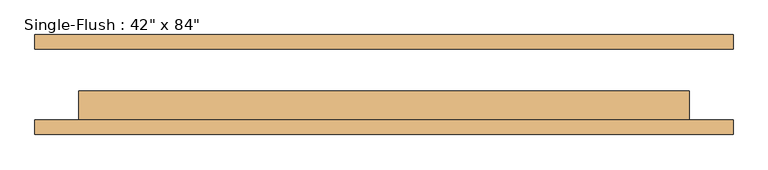
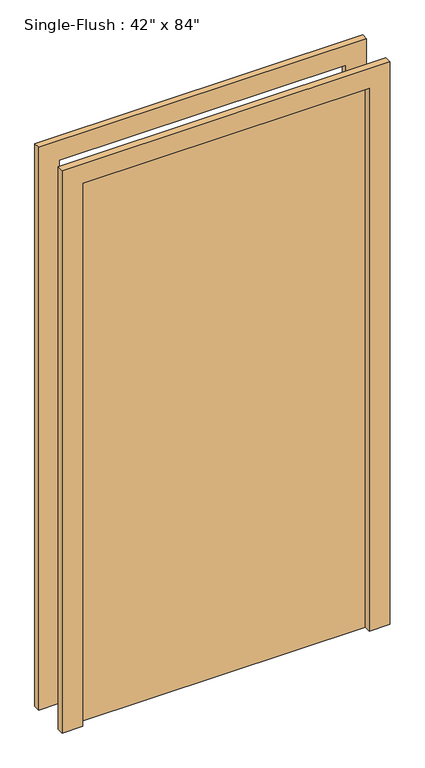
"""IFC4 building model written with IfcOpenShell, lengths in millimetres: door geometry."""

import ifcopenshell
import ifcopenshell.guid

model = None  # the IFC model being written
_history = None  # IfcOwnerHistory: only IFC2X3 demands one
_inside = {}  # id of a spatial element -> (the spatial element, [elements in it])
_under = {}  # id of a project, library or spatial element -> (it, [spatial elements below it])
_declared = {}  # id of a project -> (the project, [libraries it declares])
_typed = {}  # id of a type object -> (the type object, [elements of that type])
_made_of = {}  # id of a material, layer set ... -> (it, [elements and type objects made of it])


def new_model(schema):
    """Start an empty IFC model of exactly this schema.

    Asked for "IFC4X3", IfcOpenShell would pick the latest addendum, in which some entities
    have other attributes; the version numbers below select the first issue.
    IFC2X3 requires an IfcOwnerHistory on every rooted entity: one is made here for all.
    """
    global model, _history
    if schema == "IFC4X3":
        model = ifcopenshell.file(schema_version=(4, 3, 0, 0))
    else:
        model = ifcopenshell.file(schema=schema)
    _inside.clear()
    _under.clear()
    _declared.clear()
    _typed.clear()
    _made_of.clear()
    _history = None
    if model.schema == "IFC2X3":
        org = make("IfcOrganization", Name="unknown")
        user = make(
            "IfcPersonAndOrganization",
            ThePerson=make("IfcPerson", FamilyName="unknown"),
            TheOrganization=org,
        )
        app = make(
            "IfcApplication",
            ApplicationDeveloper=org,
            Version="unknown",
            ApplicationFullName="unknown",
            ApplicationIdentifier="unknown",
        )
        _history = make(
            "IfcOwnerHistory",
            OwningUser=user,
            OwningApplication=app,
            ChangeAction="ADDED",
            CreationDate=0,
        )
    return model


def make(cls, **values):
    """One entity of the class cls with the attributes given. An attribute that is None is left unset."""
    return model.create_entity(
        cls, **{name: value for name, value in values.items() if value is not None}
    )


def rooted(cls, **values):
    """An entity with a GlobalId (a new one), such as an element, a storey or a relation."""
    return make(cls, GlobalId=ifcopenshell.guid.new(), OwnerHistory=_history, **values)


def si_unit(unit_type, name, prefix=None):
    """IfcSIUnit, for example si_unit("LENGTHUNIT", "METRE", prefix="MILLI")."""
    return make("IfcSIUnit", UnitType=unit_type, Prefix=prefix, Name=name)


def assignment(units):
    """IfcUnitAssignment: the units of a project."""
    return None if units is None else make("IfcUnitAssignment", Units=units)


def point(xyz):
    """IfcCartesianPoint."""
    return None if xyz is None else make("IfcCartesianPoint", Coordinates=xyz)


def direction(xyz):
    """IfcDirection."""
    return None if xyz is None else make("IfcDirection", DirectionRatios=xyz)


def frame(location, z_axis=None, x_axis=None):
    """IfcAxis2Placement3D, a coordinate frame: its origin and axes. An axis left out is left unset."""
    return make(
        "IfcAxis2Placement3D",
        Location=point(location),
        Axis=direction(z_axis),
        RefDirection=direction(x_axis),
    )


def origin():
    """The frame at (0, 0, 0) with its axes left unset."""
    return frame((0.0, 0.0, 0.0))


def origin_with_axes():
    """The frame at (0, 0, 0) with the z axis (0, 0, 1) and the x axis (1, 0, 0) written out."""
    return frame((0.0, 0.0, 0.0), z_axis=(0.0, 0.0, 1.0), x_axis=(1.0, 0.0, 0.0))


def place(relative_to, where):
    """IfcLocalPlacement: puts the frame where relative to a parent placement (None: the world)."""
    return make(
        "IfcLocalPlacement", PlacementRelTo=relative_to, RelativePlacement=where
    )


def context(
    kind, dimensions, precision=None, world=None, true_north=None, identifier=None
):
    """IfcGeometricRepresentationContext, for example the 3D "Model" context."""
    return make(
        "IfcGeometricRepresentationContext",
        ContextIdentifier=identifier,
        ContextType=kind,
        CoordinateSpaceDimension=dimensions,
        Precision=precision,
        WorldCoordinateSystem=world,
        TrueNorth=true_north,
    )


def project(units=None, contexts=None):
    """IfcProject with its units and contexts."""
    return rooted(
        "IfcProject",
        Name="project",
        RepresentationContexts=contexts,
        UnitsInContext=assignment(units),
    )


def spatial(cls, under=None, at=None, **own):
    """A site, building, storey or space (cls), placed at a placement, below another one or the project."""
    s = rooted(cls, ObjectPlacement=at, **own)
    if under is not None:
        _under.setdefault(under.id(), (under, []))[1].append(s)
    return s


def polyline(points):
    """IfcPolyline through the points."""
    return make("IfcPolyline", Points=[point(p) for p in points])


def outline(outer, holes=None, kind="AREA"):
    """IfcArbitraryClosedProfileDef: a profile drawn as a closed curve; with holes, ...WithVoids."""
    if holes is None:
        return make("IfcArbitraryClosedProfileDef", ProfileType=kind, OuterCurve=outer)
    return make(
        "IfcArbitraryProfileDefWithVoids",
        ProfileType=kind,
        OuterCurve=outer,
        InnerCurves=holes,
    )


def extrude(swept, where, along, depth):
    """IfcExtrudedAreaSolid: the profile swept, set in the frame where, extruded along a direction by depth."""
    return make(
        "IfcExtrudedAreaSolid",
        SweptArea=swept,
        Position=where,
        ExtrudedDirection=direction(along),
        Depth=depth,
    )


def shape(context_of_items, identifier, shape_type, items):
    """IfcShapeRepresentation: the items that make up one representation, for example the "Body"."""
    return make(
        "IfcShapeRepresentation",
        ContextOfItems=context_of_items,
        RepresentationIdentifier=identifier,
        RepresentationType=shape_type,
        Items=items,
    )


def source(mapping_origin, context_of_items, identifier, shape_type, items):
    """IfcRepresentationMap: a shape defined once, which mapped items show again and again."""
    return make(
        "IfcRepresentationMap",
        MappingOrigin=mapping_origin,
        MappedRepresentation=shape(context_of_items, identifier, shape_type, items),
    )


def transform(
    local_origin,
    x_axis=None,
    y_axis=None,
    z_axis=None,
    scale=None,
    scale2=None,
    scale3=None,
    uniform=True,
):
    """IfcCartesianTransformationOperator3D, or its non-uniform kind. x_axis, y_axis, z_axis: its Axis1, 2, 3."""
    if uniform:
        return make(
            "IfcCartesianTransformationOperator3D",
            Axis1=direction(x_axis),
            Axis2=direction(y_axis),
            LocalOrigin=point(local_origin),
            Scale=scale,
            Axis3=direction(z_axis),
        )
    return make(
        "IfcCartesianTransformationOperator3DnonUniform",
        Axis1=direction(x_axis),
        Axis2=direction(y_axis),
        LocalOrigin=point(local_origin),
        Scale=scale,
        Axis3=direction(z_axis),
        Scale2=scale2,
        Scale3=scale3,
    )


def mapped(mapping_source, mapping_target):
    """IfcMappedItem: shows the shape of a source again, moved by a transform."""
    return make(
        "IfcMappedItem", MappingSource=mapping_source, MappingTarget=mapping_target
    )


def made_of(thing, what):
    """Note that an element or type object is made of a material, layer set ...; save() writes the relation."""
    if what is not None:
        _made_of.setdefault(what.id(), (what, []))[1].append(thing)
    return thing


def element(
    cls,
    number,
    at=None,
    inside=None,
    cuts=None,
    type_object=None,
    material=None,
    context=None,
    identifier="Body",
    shape_type=None,
    held_by="IfcProductDefinitionShape",
    body=None,
    shapes=None,
    **own,
):
    """One element of the class cls, such as IfcWall. Its Tag is "e" and its number.

    at: its placement. inside: the storey or other place that contains it. cuts: it is an
    opening in that element (IfcRelVoidsElement). A single representation is given by context,
    identifier, shape_type and body (its items); several are given by shapes. held_by: the class
    of the entity that holds the representations. save() writes the other relations.
    """
    e = rooted(cls, Tag="e%d" % number, ObjectPlacement=at, **own)
    if body is not None:
        shapes = [shape(context, identifier, shape_type, body)]
    if shapes is not None:
        e.Representation = make(held_by, Representations=shapes)
    if inside is not None:
        _inside.setdefault(inside.id(), (inside, []))[1].append(e)
    if cuts is not None:
        rooted(
            "IfcRelVoidsElement", RelatingBuildingElement=cuts, RelatedOpeningElement=e
        )
    if type_object is not None:
        _typed.setdefault(type_object.id(), (type_object, []))[1].append(e)
    return made_of(e, material)


def aggregate(whole, parts):
    """IfcRelAggregates: a whole, such as a stair, and the parts it consists of."""
    return rooted("IfcRelAggregates", RelatingObject=whole, RelatedObjects=parts)


def save(model, path):
    """Write the relations noted so far, then the file.

    IfcRelAggregates (storeys below a building ...), IfcRelContainedInSpatialStructure (elements
    in a storey), IfcRelDefinesByType, IfcRelAssociatesMaterial and IfcRelDeclares: one each for
    every whole, place, type object, material and project.
    """
    for whole, parts in _under.values():
        aggregate(whole, parts)
    for where, things in _inside.values():
        rooted(
            "IfcRelContainedInSpatialStructure",
            RelatedElements=things,
            RelatingStructure=where,
        )
    for kind, things in _typed.values():
        rooted("IfcRelDefinesByType", RelatedObjects=things, RelatingType=kind)
    for what, things in _made_of.values():
        rooted("IfcRelAssociatesMaterial", RelatedObjects=things, RelatingMaterial=what)
    for by, libraries in _declared.values():
        rooted("IfcRelDeclares", RelatingContext=by, RelatedDefinitions=libraries)
    model.write(path)


def door_8230ac15(model_context):
    return source(origin(), model_context, "Body", "SweptSolid", [
        extrude(outline(polyline([(2209.8, -609.6), (0.0, -609.6), (0.0, -533.4), (2133.6, -533.4), (2133.6, 533.4), (0.0, 533.4), (0.0, 609.6), (2209.8, 609.6), (2209.8, -609.6)])), frame((0.0, -87.3125, 0.0), z_axis=(0.0, 1.0, 0.0), x_axis=(0.0, 0.0, 1.0)), (0.0, 0.0, 1.0), 25.4),
        extrude(outline(polyline([(2209.8, 609.6), (2209.8, -609.6), (0.0, -609.6), (0.0, -533.4), (2133.6, -533.4), (2133.6, 533.4), (0.0, 533.4), (0.0, 609.6), (2209.8, 609.6)])), frame((0.0, 61.9125, 0.0), z_axis=(0.0, 1.0, 0.0), x_axis=(0.0, 0.0, 1.0)), (0.0, 0.0, 1.0), 25.4),
        extrude(outline(polyline([(533.4, -11.1125), (533.4, -61.9125), (-533.4, -61.9125), (-533.4, -11.1125), (533.4, -11.1125)])), origin_with_axes(), (0.0, 0.0, 1.0), 2133.6),
    ])


if __name__ == "__main__":
    model = new_model("IFC4")
    model_context = context("Model", 3, world=origin())
    ifc_project = project(units=[si_unit("LENGTHUNIT", "METRE", prefix="MILLI")], contexts=[model_context])
    site = spatial("IfcSite", under=ifc_project)
    building = spatial("IfcBuilding", under=site)
    placement = place(None, origin())
    door_shape = door_8230ac15(model_context)
    element("IfcDoor", 1, ObjectType="Single-Flush : 42\" x 84\"", at=placement, inside=building, context=model_context, shape_type="MappedRepresentation", body=[
        mapped(door_shape, transform((0.0, 0.0, 0.0), x_axis=(1.0, 0.0, 0.0), y_axis=(0.0, 1.0, 0.0), z_axis=(0.0, 0.0, 1.0))),
    ])
    save(model, "model.ifc")

# Revit data of these elements
# Type "Single-Flush : 42\" x 84\""
#   Type Mark = "9"
#   Construction Type = "B"
#   Assembly Code = "C1020"
#   Thickness = 0' - 2"
#   Height = 7' - 0"
#   Trim Projection Ext = 0' - 1"
#   Trim Projection Int = 0' - 1"
#   Trim Width = 0' - 3"
#   Width = 3' - 6"
#   Door Material = Door - Panel
#   Frame Material = Door - Frame
#   Function = (empty or 0)
#   Wall Closure = (empty or 0)
# Element 1 (IfcDoor, "Single-Flush : 42\" x 84\"")
#   Materials on its faces: "Door - Frame", "Door - Panel"
# Materials
#   "Door - Panel": class "Wood", colour RGB 210 159 95, transparency 0
#   "Door - Frame": class "Miscellaneous", colour RGB 118 70 51, transparency 0
